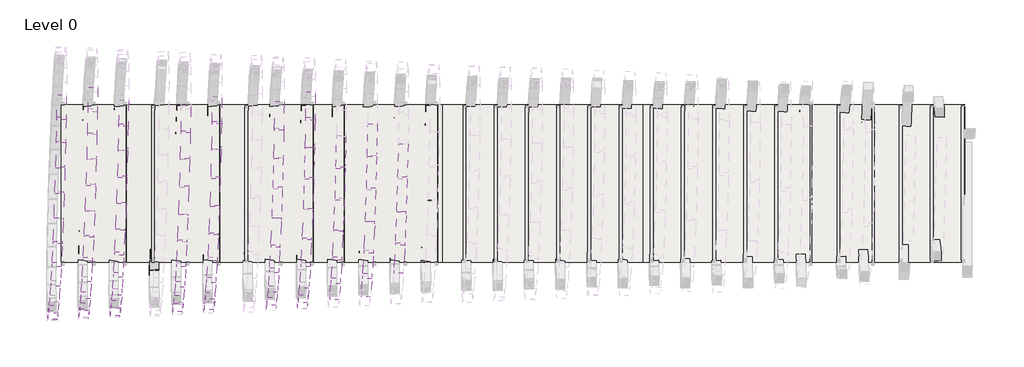
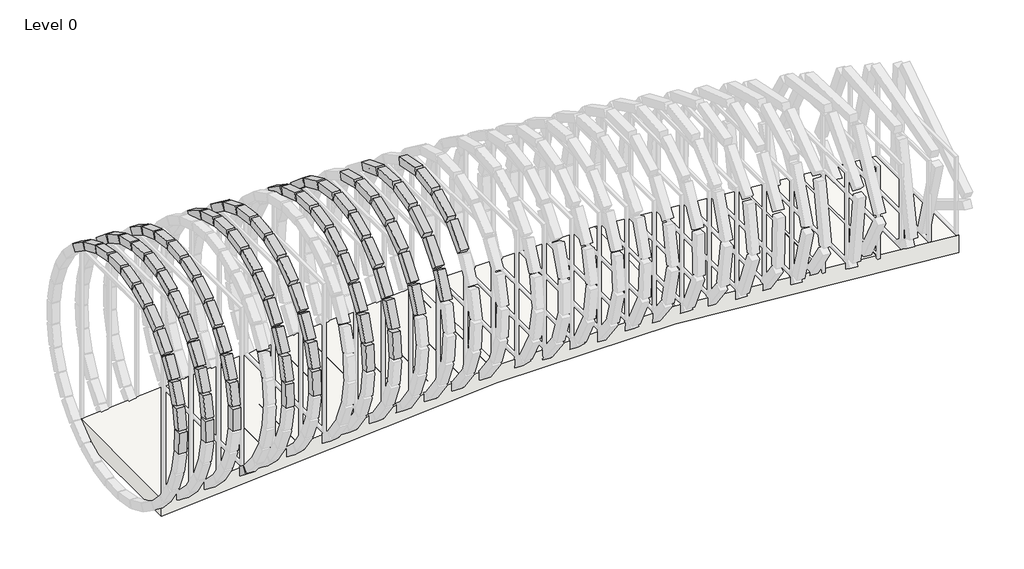
# One storey, part 1 of 6: 94 proxies, 1 slab.
"""IFC4 building model written with IfcOpenShell, lengths in millimetres."""

import ifcopenshell
import ifcopenshell.guid

model = None  # the IFC model being written
_history = None  # IfcOwnerHistory: only IFC2X3 demands one
_inside = {}  # id of a spatial element -> (the spatial element, [elements in it])
_under = {}  # id of a project, library or spatial element -> (it, [spatial elements below it])
_declared = {}  # id of a project -> (the project, [libraries it declares])
_typed = {}  # id of a type object -> (the type object, [elements of that type])
_made_of = {}  # id of a material, layer set ... -> (it, [elements and type objects made of it])


def new_model(schema):
    """Start an empty IFC model of exactly this schema.

    Asked for "IFC4X3", IfcOpenShell would pick the latest addendum, in which some entities
    have other attributes; the version numbers below select the first issue.
    IFC2X3 requires an IfcOwnerHistory on every rooted entity: one is made here for all.
    """
    global model, _history
    if schema == "IFC4X3":
        model = ifcopenshell.file(schema_version=(4, 3, 0, 0))
    else:
        model = ifcopenshell.file(schema=schema)
    _inside.clear()
    _under.clear()
    _declared.clear()
    _typed.clear()
    _made_of.clear()
    _history = None
    if model.schema == "IFC2X3":
        org = make("IfcOrganization", Name="unknown")
        user = make(
            "IfcPersonAndOrganization",
            ThePerson=make("IfcPerson", FamilyName="unknown"),
            TheOrganization=org,
        )
        app = make(
            "IfcApplication",
            ApplicationDeveloper=org,
            Version="unknown",
            ApplicationFullName="unknown",
            ApplicationIdentifier="unknown",
        )
        _history = make(
            "IfcOwnerHistory",
            OwningUser=user,
            OwningApplication=app,
            ChangeAction="ADDED",
            CreationDate=0,
        )
    return model


def make(cls, **values):
    """One entity of the class cls with the attributes given. An attribute that is None is left unset."""
    return model.create_entity(
        cls, **{name: value for name, value in values.items() if value is not None}
    )


def rooted(cls, **values):
    """An entity with a GlobalId (a new one), such as an element, a storey or a relation."""
    return make(cls, GlobalId=ifcopenshell.guid.new(), OwnerHistory=_history, **values)


def si_unit(unit_type, name, prefix=None):
    """IfcSIUnit, for example si_unit("LENGTHUNIT", "METRE", prefix="MILLI")."""
    return make("IfcSIUnit", UnitType=unit_type, Prefix=prefix, Name=name)


def assignment(units):
    """IfcUnitAssignment: the units of a project."""
    return None if units is None else make("IfcUnitAssignment", Units=units)


def point(xyz):
    """IfcCartesianPoint."""
    return None if xyz is None else make("IfcCartesianPoint", Coordinates=xyz)


def direction(xyz):
    """IfcDirection."""
    return None if xyz is None else make("IfcDirection", DirectionRatios=xyz)


def frame(location, z_axis=None, x_axis=None):
    """IfcAxis2Placement3D, a coordinate frame: its origin and axes. An axis left out is left unset."""
    return make(
        "IfcAxis2Placement3D",
        Location=point(location),
        Axis=direction(z_axis),
        RefDirection=direction(x_axis),
    )


def origin():
    """The frame at (0, 0, 0) with its axes left unset."""
    return frame((0.0, 0.0, 0.0))


def place(relative_to, where):
    """IfcLocalPlacement: puts the frame where relative to a parent placement (None: the world)."""
    return make(
        "IfcLocalPlacement", PlacementRelTo=relative_to, RelativePlacement=where
    )


def context(
    kind, dimensions, precision=None, world=None, true_north=None, identifier=None
):
    """IfcGeometricRepresentationContext, for example the 3D "Model" context."""
    return make(
        "IfcGeometricRepresentationContext",
        ContextIdentifier=identifier,
        ContextType=kind,
        CoordinateSpaceDimension=dimensions,
        Precision=precision,
        WorldCoordinateSystem=world,
        TrueNorth=true_north,
    )


def project(units=None, contexts=None):
    """IfcProject with its units and contexts."""
    return rooted(
        "IfcProject",
        Name="project",
        RepresentationContexts=contexts,
        UnitsInContext=assignment(units),
    )


def spatial(cls, under=None, at=None, **own):
    """A site, building, storey or space (cls), placed at a placement, below another one or the project."""
    s = rooted(cls, ObjectPlacement=at, **own)
    if under is not None:
        _under.setdefault(under.id(), (under, []))[1].append(s)
    return s


def polyline(points):
    """IfcPolyline through the points."""
    return make("IfcPolyline", Points=[point(p) for p in points])


def outline(outer, holes=None, kind="AREA"):
    """IfcArbitraryClosedProfileDef: a profile drawn as a closed curve; with holes, ...WithVoids."""
    if holes is None:
        return make("IfcArbitraryClosedProfileDef", ProfileType=kind, OuterCurve=outer)
    return make(
        "IfcArbitraryProfileDefWithVoids",
        ProfileType=kind,
        OuterCurve=outer,
        InnerCurves=holes,
    )


def extrude(swept, where, along, depth):
    """IfcExtrudedAreaSolid: the profile swept, set in the frame where, extruded along a direction by depth."""
    return make(
        "IfcExtrudedAreaSolid",
        SweptArea=swept,
        Position=where,
        ExtrudedDirection=direction(along),
        Depth=depth,
    )


def faces_of(points, faces, orient=None, outer=None):
    """IfcFace entities. A face is a list of loops; a loop is a list of indices into points, from 0.

    orient and outer hold one flag for each loop. By default every Orientation is true, the
    first loop of a face is its IfcFaceOuterBound and the others are IfcFaceBound.
    """
    made = []
    for i, loops in enumerate(faces):
        bounds = []
        for j, loop in enumerate(loops):
            is_outer = j == 0 if outer is None else outer[i][j]
            bounds.append(
                make(
                    "IfcFaceOuterBound" if is_outer else "IfcFaceBound",
                    Bound=make("IfcPolyLoop", Polygon=[points[k] for k in loop]),
                    Orientation=True if orient is None else orient[i][j],
                )
            )
        made.append(make("IfcFace", Bounds=bounds))
    return made


def faceted_brep(points, faces, orient=None, outer=None, voids=None):
    """IfcFacetedBrep: a solid bounded by flat faces; with voids (closed shells), ...WithVoids."""
    shared = [point(p) for p in points]
    hull = make("IfcClosedShell", CfsFaces=faces_of(shared, faces, orient, outer))
    if voids is None:
        return make("IfcFacetedBrep", Outer=hull)
    return make(
        "IfcFacetedBrepWithVoids",
        Outer=hull,
        Voids=[
            make(cls, CfsFaces=faces_of(shared, fs, o, b)) for cls, fs, o, b in voids
        ],
    )


def shape(context_of_items, identifier, shape_type, items):
    """IfcShapeRepresentation: the items that make up one representation, for example the "Body"."""
    return make(
        "IfcShapeRepresentation",
        ContextOfItems=context_of_items,
        RepresentationIdentifier=identifier,
        RepresentationType=shape_type,
        Items=items,
    )


def source(mapping_origin, context_of_items, identifier, shape_type, items):
    """IfcRepresentationMap: a shape defined once, which mapped items show again and again."""
    return make(
        "IfcRepresentationMap",
        MappingOrigin=mapping_origin,
        MappedRepresentation=shape(context_of_items, identifier, shape_type, items),
    )


def transform(
    local_origin,
    x_axis=None,
    y_axis=None,
    z_axis=None,
    scale=None,
    scale2=None,
    scale3=None,
    uniform=True,
):
    """IfcCartesianTransformationOperator3D, or its non-uniform kind. x_axis, y_axis, z_axis: its Axis1, 2, 3."""
    if uniform:
        return make(
            "IfcCartesianTransformationOperator3D",
            Axis1=direction(x_axis),
            Axis2=direction(y_axis),
            LocalOrigin=point(local_origin),
            Scale=scale,
            Axis3=direction(z_axis),
        )
    return make(
        "IfcCartesianTransformationOperator3DnonUniform",
        Axis1=direction(x_axis),
        Axis2=direction(y_axis),
        LocalOrigin=point(local_origin),
        Scale=scale,
        Axis3=direction(z_axis),
        Scale2=scale2,
        Scale3=scale3,
    )


def mapped(mapping_source, mapping_target):
    """IfcMappedItem: shows the shape of a source again, moved by a transform."""
    return make(
        "IfcMappedItem", MappingSource=mapping_source, MappingTarget=mapping_target
    )


def made_of(thing, what):
    """Note that an element or type object is made of a material, layer set ...; save() writes the relation."""
    if what is not None:
        _made_of.setdefault(what.id(), (what, []))[1].append(thing)
    return thing


def element(
    cls,
    number,
    at=None,
    inside=None,
    cuts=None,
    type_object=None,
    material=None,
    context=None,
    identifier="Body",
    shape_type=None,
    held_by="IfcProductDefinitionShape",
    body=None,
    shapes=None,
    **own,
):
    """One element of the class cls, such as IfcWall. Its Tag is "e" and its number.

    at: its placement. inside: the storey or other place that contains it. cuts: it is an
    opening in that element (IfcRelVoidsElement). A single representation is given by context,
    identifier, shape_type and body (its items); several are given by shapes. held_by: the class
    of the entity that holds the representations. save() writes the other relations.
    """
    e = rooted(cls, Tag="e%d" % number, ObjectPlacement=at, **own)
    if body is not None:
        shapes = [shape(context, identifier, shape_type, body)]
    if shapes is not None:
        e.Representation = make(held_by, Representations=shapes)
    if inside is not None:
        _inside.setdefault(inside.id(), (inside, []))[1].append(e)
    if cuts is not None:
        rooted(
            "IfcRelVoidsElement", RelatingBuildingElement=cuts, RelatedOpeningElement=e
        )
    if type_object is not None:
        _typed.setdefault(type_object.id(), (type_object, []))[1].append(e)
    return made_of(e, material)


def aggregate(whole, parts):
    """IfcRelAggregates: a whole, such as a stair, and the parts it consists of."""
    return rooted("IfcRelAggregates", RelatingObject=whole, RelatedObjects=parts)


def save(model, path):
    """Write the relations noted so far, then the file.

    IfcRelAggregates (storeys below a building ...), IfcRelContainedInSpatialStructure (elements
    in a storey), IfcRelDefinesByType, IfcRelAssociatesMaterial and IfcRelDeclares: one each for
    every whole, place, type object, material and project.
    """
    for whole, parts in _under.values():
        aggregate(whole, parts)
    for where, things in _inside.values():
        rooted(
            "IfcRelContainedInSpatialStructure",
            RelatedElements=things,
            RelatingStructure=where,
        )
    for kind, things in _typed.values():
        rooted("IfcRelDefinesByType", RelatedObjects=things, RelatingType=kind)
    for what, things in _made_of.values():
        rooted("IfcRelAssociatesMaterial", RelatedObjects=things, RelatingMaterial=what)
    for by, libraries in _declared.values():
        rooted("IfcRelDeclares", RelatingContext=by, RelatedDefinitions=libraries)
    model.write(path)


def family2_family2_c0c01265(model_context):
    return source(origin(), model_context, "Body", "Brep", [
        faceted_brep([(-3947.6024006, -6432.4470029, 1.0945136), (-3947.6024006, -6432.4470029, 201.0945136), (-3939.2403939, -5715.1531197, 202.060409), (-3939.2403939, -5715.1531197, 2.060409), (-3747.6112106, -6434.3242155, 201.0945136), (-3739.249204, -5717.0303324, 202.060409), (-3747.6112106, -6434.3242155, 1.0945136), (-3739.249204, -5717.0303324, 2.060409)], [[[0, 1, 2, 3]], [[1, 4, 5, 2]], [[4, 6, 7, 5]], [[6, 0, 3, 7]], [[3, 2, 5, 7]], [[0, 6, 4, 1]]]),
    ])


def family2_family2_390b1421(model_context):
    return source(origin(), model_context, "Body", "Brep", [
        faceted_brep([(-3947.4886476, -6420.3281868, 1.0945136), (-3947.4886476, -6420.3281868, 201.0945136), (-3939.3541469, -5727.2719358, 202.060409), (-3939.3541469, -5727.2719358, 2.060409), (-3747.4974576, -6422.2053995, 201.0945136), (-3739.3629569, -5729.1491484, 202.060409), (-3747.4974576, -6422.2053995, 1.0945136), (-3739.3629569, -5729.1491484, 2.060409)], [[[0, 1, 2, 3]], [[1, 4, 5, 2]], [[4, 6, 7, 5]], [[6, 0, 3, 7]], [[3, 2, 5, 7]], [[0, 6, 4, 1]]]),
    ])


def family2_family2_5d0bf995(model_context):
    return source(origin(), model_context, "Body", "Brep", [
        faceted_brep([(-3947.3850716, -6409.2935888, 1.0945136), (-3947.3850716, -6409.2935888, 201.0945136), (-3939.4577229, -5738.3065338, 202.060409), (-3939.4577229, -5738.3065338, 2.060409), (-3747.3938816, -6411.1708015, 201.0945136), (-3739.4665329, -5740.1837465, 202.060409), (-3747.3938816, -6411.1708015, 1.0945136), (-3739.4665329, -5740.1837465, 2.060409)], [[[0, 1, 2, 3]], [[1, 4, 5, 2]], [[4, 6, 7, 5]], [[6, 0, 3, 7]], [[3, 2, 5, 7]], [[0, 6, 4, 1]]]),
    ])


def family2_family2_428b8be4(model_context):
    return source(origin(), model_context, "Body", "Brep", [
        faceted_brep([(-3947.2904042, -6399.2080776, 1.0945136), (-3947.2904042, -6399.2080776, 201.0945136), (-3939.5523903, -5748.392045, 202.060409), (-3939.5523903, -5748.392045, 2.060409), (-3747.2992142, -6401.0852903, 201.0945136), (-3739.5612004, -5750.2692577, 202.060409), (-3747.2992142, -6401.0852903, 1.0945136), (-3739.5612004, -5750.2692577, 2.060409)], [[[0, 1, 2, 3]], [[1, 4, 5, 2]], [[4, 6, 7, 5]], [[6, 0, 3, 7]], [[3, 2, 5, 7]], [[0, 6, 4, 1]]]),
    ])


def family2_family2_042d18f2(model_context):
    return source(origin(), model_context, "Body", "Brep", [
        faceted_brep([(-3947.2035772, -6389.957857, 1.0945136), (-3947.2035772, -6389.957857, 201.0945136), (-3939.6392173, -5757.6422656, 202.060409), (-3939.6392173, -5757.6422656, 2.060409), (-3747.2123872, -6391.8350697, 201.0945136), (-3739.6480273, -5759.5194783, 202.060409), (-3747.2123872, -6391.8350697, 1.0945136), (-3739.6480273, -5759.5194783, 2.060409)], [[[0, 1, 2, 3]], [[1, 4, 5, 2]], [[4, 6, 7, 5]], [[6, 0, 3, 7]], [[3, 2, 5, 7]], [[0, 6, 4, 1]]]),
    ])


def family2_family2_49637704(model_context):
    return source(origin(), model_context, "Body", "Brep", [
        faceted_brep([(-3947.1236849, -6381.446434, 1.0945136), (-3947.1236849, -6381.446434, 201.0945136), (-3939.7191096, -5766.1536886, 202.060409), (-3939.7191096, -5766.1536886, 2.060409), (-3747.1324949, -6383.3236466, 201.0945136), (-3739.7279196, -5768.0309013, 202.060409), (-3747.1324949, -6383.3236466, 1.0945136), (-3739.7279196, -5768.0309013, 2.060409)], [[[0, 1, 2, 3]], [[1, 4, 5, 2]], [[4, 6, 7, 5]], [[6, 0, 3, 7]], [[3, 2, 5, 7]], [[0, 6, 4, 1]]]),
    ])


def family2_family2_4fb73a58(model_context):
    return source(origin(), model_context, "Body", "Brep", [
        faceted_brep([(-3947.0499544, -6373.591465, 1.0945136), (-3947.0499544, -6373.591465, 201.0945136), (-3939.7928401, -5774.0086576, 202.060409), (-3939.7928401, -5774.0086576, 2.060409), (-3747.0587644, -6375.4686776, 201.0945136), (-3739.8016501, -5775.8858703, 202.060409), (-3747.0587644, -6375.4686776, 1.0945136), (-3739.8016501, -5775.8858703, 2.060409)], [[[0, 1, 2, 3]], [[1, 4, 5, 2]], [[4, 6, 7, 5]], [[6, 0, 3, 7]], [[3, 2, 5, 7]], [[0, 6, 4, 1]]]),
    ])


def family2_family2_6873a2fb(model_context):
    return source(origin(), model_context, "Body", "Brep", [
        faceted_brep([(-3946.9817223, -6366.3222661, 1.0945136), (-3946.9817223, -6366.3222661, 201.0945136), (-3939.8610722, -5781.2778565, 202.060409), (-3939.8610722, -5781.2778565, 2.060409), (-3746.9905323, -6368.1994787, 201.0945136), (-3739.8698823, -5783.1550692, 202.060409), (-3746.9905323, -6368.1994787, 1.0945136), (-3739.8698823, -5783.1550692, 2.060409)], [[[0, 1, 2, 3]], [[1, 4, 5, 2]], [[4, 6, 7, 5]], [[6, 0, 3, 7]], [[3, 2, 5, 7]], [[0, 6, 4, 1]]]),
    ])


def family2_family2_2698309a(model_context):
    return source(origin(), model_context, "Body", "Brep", [
        faceted_brep([(-3946.9184158, -6359.5778294, 1.0945136), (-3946.9184158, -6359.5778294, 201.0945136), (-3939.9243787, -5788.0222932, 202.060409), (-3939.9243787, -5788.0222932, 2.060409), (-3746.9272258, -6361.4550421, 201.0945136), (-3739.9331888, -5789.8995058, 202.060409), (-3746.9272258, -6361.4550421, 1.0945136), (-3739.9331888, -5789.8995058, 2.060409)], [[[0, 1, 2, 3]], [[1, 4, 5, 2]], [[4, 6, 7, 5]], [[6, 0, 3, 7]], [[3, 2, 5, 7]], [[0, 6, 4, 1]]]),
    ])


def family2_family2_b00769dc(model_context):
    return source(origin(), model_context, "Body", "Brep", [
        faceted_brep([(-3946.8595382, -6353.3052302, 1.0945136), (-3946.8595382, -6353.3052302, 201.0945136), (-3939.9832564, -5794.2948924, 202.060409), (-3939.9832564, -5794.2948924, 2.060409), (-3746.8683482, -6355.1824428, 201.0945136), (-3739.9920664, -5796.1721051, 202.060409), (-3746.8683482, -6355.1824428, 1.0945136), (-3739.9920664, -5796.1721051, 2.060409)], [[[0, 1, 2, 3]], [[1, 4, 5, 2]], [[4, 6, 7, 5]], [[6, 0, 3, 7]], [[3, 2, 5, 7]], [[0, 6, 4, 1]]]),
    ])


def family2_family2_2f13623d(model_context):
    return source(origin(), model_context, "Body", "Brep", [
        faceted_brep([(-3946.8046564, -6347.4583376, 1.0945136), (-3946.8046564, -6347.4583376, 201.0945136), (-3940.0381381, -5800.141785, 202.060409), (-3940.0381381, -5800.141785, 2.060409), (-3746.8134664, -6349.3355503, 201.0945136), (-3740.0469481, -5802.0189977, 202.060409), (-3746.8134664, -6349.3355503, 1.0945136), (-3740.0469481, -5802.0189977, 2.060409)], [[[0, 1, 2, 3]], [[1, 4, 5, 2]], [[4, 6, 7, 5]], [[6, 0, 3, 7]], [[3, 2, 5, 7]], [[0, 6, 4, 1]]]),
    ])


def family2_family2_c4a0287a(model_context):
    return source(origin(), model_context, "Body", "Brep", [
        faceted_brep([(-3946.7533915, -6341.9967642, 1.0945136), (-3946.7533915, -6341.9967642, 201.0945136), (-3940.089403, -5805.6033584, 202.060409), (-3940.089403, -5805.6033584, 2.060409), (-3746.7622015, -6343.8739769, 201.0945136), (-3740.098213, -5807.480571, 202.060409), (-3746.7622015, -6343.8739769, 1.0945136), (-3740.098213, -5807.480571, 2.060409)], [[[0, 1, 2, 3]], [[1, 4, 5, 2]], [[4, 6, 7, 5]], [[6, 0, 3, 7]], [[3, 2, 5, 7]], [[0, 6, 4, 1]]]),
    ])


model = new_model("IFC4")

# Units and contexts
model_context = context("Model", 3, world=origin())
ifc_project = project(units=[si_unit("LENGTHUNIT", "METRE", prefix="MILLI")], contexts=[model_context])

# Site, building, storey
site = spatial("IfcSite", under=ifc_project)
building = spatial("IfcBuilding", under=site)
storey = spatial("IfcBuildingStorey", under=building, Name="Level 0", Elevation=0.0)

# Proxies
placement = place(None, origin())
family2_family2_shape = family2_family2_c0c01265(model_context)
element("IfcBuildingElementProxy", 1, Name="Family2 : Family2", ObjectType="Family2 : Family2", at=placement, inside=storey, context=model_context, shape_type="MappedRepresentation", body=[
    mapped(family2_family2_shape, transform((-6396.5684291, -2837.5092631, 6085.2878101), x_axis=(-0.9993635970569693, 0.019515115875459933, 0.029859020910323705), y_axis=(-0.013210966255060963, -0.9800389734063266, 0.1983660277751243), z_axis=(0.03313414021765793, 0.19784532053359544, 0.9796730872566602))),
])
element("IfcBuildingElementProxy", 2, Name="Family2 : Family2", ObjectType="Family2 : Family2", at=placement, inside=storey, context=model_context, shape_type="MappedRepresentation", body=[
    mapped(family2_family2_shape, transform((-6470.2682928, -3665.5268728, 4304.1033014), x_axis=(-0.9994458455142355, 0.019376337243089063, 0.02706583527950426), y_axis=(-0.021973408141946323, -0.9948239279417687, -0.09920948406850226), z_axis=(0.025003424144757144, -0.09974923533317458, 0.994698405966092))),
])
element("IfcBuildingElementProxy", 3, Name="Family2 : Family2", ObjectType="Family2 : Family2", at=placement, inside=storey, context=model_context, shape_type="MappedRepresentation", body=[
    mapped(family2_family2_shape, transform((-6532.4519203, -3931.5588011, 2357.5619339), x_axis=(-0.999501945539641, 0.020067046494086277, 0.02435517414179686), y_axis=(-0.02795009425626786, -0.9212383571752715, -0.3879931462024461), z_axis=(0.014651044110875288, -0.38848063389828225, 0.9213404061433809))),
])
element("IfcBuildingElementProxy", 4, Name="Family2 : Family2", ObjectType="Family2 : Family2", at=placement, inside=storey, context=model_context, shape_type="MappedRepresentation", body=[
    mapped(family2_family2_shape, transform((-6577.5940234, -3611.9669438, 418.6224503), x_axis=(-0.9995269123997371, 0.02152587108037278, 0.021967891634827073), y_axis=(-0.030609969808513042, -0.7658206619943964, -0.6423252629398807), z_axis=(0.002996854512694002, -0.6426938233223469, 0.7661172679990537))),
])
family2_family2_2_shape = family2_family2_390b1421(model_context)
element("IfcBuildingElementProxy", 5, Name="Family2 : Family2", ObjectType="Family2 : Family2", at=placement, inside=storey, context=model_context, shape_type="MappedRepresentation", body=[
    mapped(family2_family2_2_shape, transform((-7043.8373064, -2077.9606819, 7037.3849212), x_axis=(-0.9993079250855319, 0.020318015980282017, 0.03115845130738213), y_axis=(-0.007279883403612856, -0.9282706726012948, 0.371834051272836), z_axis=(0.03647840674809277, 0.3713498843610499, 0.92777615254228))),
])
element("IfcBuildingElementProxy", 6, Name="Family2 : Family2", ObjectType="Family2 : Family2", at=placement, inside=storey, context=model_context, shape_type="MappedRepresentation", body=[
    mapped(family2_family2_2_shape, transform((-7118.0067992, -3181.769788, 5516.9346303), x_axis=(-0.9993980532845504, 0.019688875205587705, 0.028563600686710367), y_axis=(-0.016881803397264153, -0.9952969690227281, 0.09538840688588489), z_axis=(0.03030735562709434, 0.09484878305655688, 0.9950302370016618))),
])
element("IfcBuildingElementProxy", 7, Name="Family2 : Family2", ObjectType="Family2 : Family2", at=placement, inside=storey, context=model_context, shape_type="MappedRepresentation", body=[
    mapped(family2_family2_2_shape, transform((-7185.3404976, -3812.2729758, 3746.7378484), x_axis=(-0.9994682121798837, 0.019816387397900603, 0.025896015763889266), y_axis=(-0.0243562687384851, -0.9817122987182729, -0.18880607701666632), z_axis=(0.02168098279797224, -0.18933640256374623, 0.9816728893318453))),
])
element("IfcBuildingElementProxy", 8, Name="Family2 : Family2", ObjectType="Family2 : Family2", at=placement, inside=storey, context=model_context, shape_type="MappedRepresentation", body=[
    mapped(family2_family2_2_shape, transform((-7240.3834258, -3918.3906269, 1870.205391), x_axis=(-0.9995127179150824, 0.020690222277743867, 0.02337180840462852), y_axis=(-0.029097742697687057, -0.8886172108848517, -0.457725653518706), z_axis=(0.011298145684328523, -0.45818267887527653, 0.8887862424018338))),
])
element("IfcBuildingElementProxy", 9, Name="Family2 : Family2", ObjectType="Family2 : Family2", at=placement, inside=storey, context=model_context, shape_type="MappedRepresentation", body=[
    mapped(family2_family2_2_shape, transform((-7278.6763332, -3491.5257202, 39.3627577), x_axis=(-0.9995279649001668, 0.02223958694004874, 0.021195474877135474), y_axis=(-0.030722099253326866, -0.7235537158809213, -0.6895840578583441), z_axis=(0.0, -0.6899097194616461, 0.7238954199277359))),
])
element("IfcBuildingElementProxy", 10, Name="Family2 : Family2", ObjectType="Family2 : Family2", at=placement, inside=storey, context=model_context, shape_type="MappedRepresentation", body=[
    mapped(family2_family2_2_shape, transform((-7297.1169561, -2566.2603118, -1597.4660699), x_axis=(-0.9995127179150824, 0.02433896107430176, 0.019543328780653933), y_axis=(-0.029097742697686946, -0.49989427640129913, -0.8655975010310053), z_axis=(-0.011298145684328832, -0.865744377628319, 0.5003588957029249))),
])
family2_family2_3_shape = family2_family2_5d0bf995(model_context)
element("IfcBuildingElementProxy", 11, Name="Family2 : Family2", ObjectType="Family2 : Family2", at=placement, inside=storey, context=model_context, shape_type="MappedRepresentation", body=[
    mapped(family2_family2_3_shape, transform((-7766.7940735, -2531.5035471, 6528.1339417), x_axis=(-0.9993471346343662, 0.020301994662961675, 0.02988533939555133), y_axis=(-0.011457121548771567, -0.9625718139560835, 0.27078448504874103), z_axis=(0.03426425052294141, 0.27026529927092063, 0.9621759865773523))),
])
element("IfcBuildingElementProxy", 12, Name="Family2 : Family2", ObjectType="Family2 : Family2", at=placement, inside=storey, context=model_context, shape_type="MappedRepresentation", body=[
    mapped(family2_family2_3_shape, transform((-7836.0862349, -3444.6813187, 4975.6904694), x_axis=(-0.9994266506244945, 0.019952546178124225, 0.027354449775399966), y_axis=(-0.019928456644108153, -0.9998007437454588, 0.0011530055558309493), z_axis=(0.027372004626789022, 0.0006072125144431367, 0.9996251320648525))),
])
element("IfcBuildingElementProxy", 13, Name="Family2 : Family2", ObjectType="Family2 : Family2", at=placement, inside=storey, context=model_context, shape_type="MappedRepresentation", body=[
    mapped(family2_family2_3_shape, transform((-7897.2581176, -3904.9775123, 3234.0931577), x_axis=(-0.9994857645079068, 0.02029891933854758, 0.024822578829211326), y_axis=(-0.02622622787686343, -0.9628994474747761, -0.2685830207293869), z_axis=(0.01844970236605738, -0.2690959084164204, 0.9629366544877943))),
])
element("IfcBuildingElementProxy", 14, Name="Family2 : Family2", ObjectType="Family2 : Family2", at=placement, inside=storey, context=model_context, shape_type="MappedRepresentation", body=[
    mapped(family2_family2_3_shape, transform((-7945.772883, -3878.254065, 1432.5083121), x_axis=(-0.9995200920782988, 0.02131542523147494, 0.022477503842524255), y_axis=(-0.02988335836509007, -0.8546047254762345, -0.5184185066975466), z_axis=(0.008159070082607002, -0.5188414168519047, 0.8548315703894513))),
])
element("IfcBuildingElementProxy", 15, Name="Family2 : Family2", ObjectType="Family2 : Family2", at=placement, inside=storey, context=model_context, shape_type="MappedRepresentation", body=[
    mapped(family2_family2_3_shape, transform((-7978.0324128, -3366.4929326, -295.4487611), x_axis=(-0.9995270874168127, 0.022926674265032795, 0.02049314829909779), y_axis=(-0.03062861547073516, -0.6829483018650779, -0.7298242972756885), z_axis=(-0.002736683103608129, -0.7301068309410284, 0.6833275393095458))),
])
element("IfcBuildingElementProxy", 16, Name="Family2 : Family2", ObjectType="Family2 : Family2", at=placement, inside=storey, context=model_context, shape_type="MappedRepresentation", body=[
    mapped(family2_family2_3_shape, transform((-7991.6441653, -2407.6490971, -1821.6233908), x_axis=(-0.999506231711192, 0.025013167469376377, 0.019016682771764888), y_axis=(-0.02840672688359737, -0.46066114830466015, -0.8871213920937727), z_axis=(-0.013429469023521176, -0.887223561395763, 0.46114423065453763))),
])
family2_family2_4_shape = family2_family2_428b8be4(model_context)
element("IfcBuildingElementProxy", 17, Name="Family2 : Family2", ObjectType="Family2 : Family2", at=placement, inside=storey, context=model_context, shape_type="MappedRepresentation", body=[
    mapped(family2_family2_4_shape, transform((-8349.1757108, -349.9613425, 8322.8659908), x_axis=(-0.9992006919462781, 0.022454860439543138, 0.033071989004595945), y_axis=(0.0041443327129058564, -0.7646748671158883, 0.6444029578669418), z_axis=(0.03975929728307849, 0.644024942718789, 0.7639705959234404))),
])
element("IfcBuildingElementProxy", 18, Name="Family2 : Family2", ObjectType="Family2 : Family2", at=placement, inside=storey, context=model_context, shape_type="MappedRepresentation", body=[
    mapped(family2_family2_4_shape, transform((-8417.9429112, -1775.2827593, 7343.0038201), x_axis=(-0.9992956048051683, 0.021134817771098994, 0.03100989672435847), y_axis=(-0.005967326982465977, -0.9053072577395126, 0.42471538716280155), z_axis=(0.037049766878582024, 0.4242311734914662, 0.9047956820256695))),
])
element("IfcBuildingElementProxy", 19, Name="Family2 : Family2", ObjectType="Family2 : Family2", at=placement, inside=storey, context=model_context, shape_type="MappedRepresentation", body=[
    mapped(family2_family2_4_shape, transform((-8486.820728, -2898.1535958, 6027.3986842), x_axis=(-0.9993807013464429, 0.020393697698042258, 0.028675963287971513), y_axis=(-0.015033193048246478, -0.9842634082524215, 0.17606688013962607), z_axis=(0.03181535608894513, 0.17552675086586705, 0.9839604376434075))),
])
element("IfcBuildingElementProxy", 20, Name="Family2 : Family2", ObjectType="Family2 : Family2", at=placement, inside=storey, context=model_context, shape_type="MappedRepresentation", body=[
    mapped(family2_family2_4_shape, transform((-8551.115252, -3642.0520602, 4465.7068992), x_axis=(-0.9994501823814422, 0.020282006328592724, 0.02622924240211747), y_axis=(-0.022435441694104982, -0.9961625874783727, -0.08459757836004667), z_axis=(0.024412781359208695, -0.08513952975957023, 0.9960699155072533))),
])
element("IfcBuildingElementProxy", 21, Name="Family2 : Family2", ObjectType="Family2 : Family2", at=placement, inside=storey, context=model_context, shape_type="MappedRepresentation", body=[
    mapped(family2_family2_4_shape, transform((-8606.4449175, -3956.2827014, 2764.3551793), x_axis=(-0.9994993128924541, 0.020807355244999624, 0.023836474051769297), y_axis=(-0.02766962190762047, -0.9401938860174409, -0.33951413625784876), z_axis=(0.015346515923870596, -0.3400036921316182, 0.940298874712645))),
])
element("IfcBuildingElementProxy", 22, Name="Family2 : Family2", ObjectType="Family2 : Family2", at=placement, inside=storey, context=model_context, shape_type="MappedRepresentation", body=[
    mapped(family2_family2_4_shape, transform((-8649.0390993, -3819.4312207, 1039.2878327), x_axis=(-0.9995247447163452, 0.021933942786790245, 0.021660721445766612), y_axis=(-0.030379032957133623, -0.820171478381537, -0.5713106514025741), z_axis=(0.005234410789637128, -0.571697164767563, 0.8204480195237328))),
])
element("IfcBuildingElementProxy", 23, Name="Family2 : Family2", ObjectType="Family2 : Family2", at=placement, inside=storey, context=model_context, shape_type="MappedRepresentation", body=[
    mapped(family2_family2_4_shape, transform((-8675.9950743, -3240.8238202, -591.9346519), x_axis=(-0.9995247447163452, 0.023584993874764825, 0.019850258528608347), y_axis=(-0.03037903295713377, -0.6442746933046386, -0.7641905743489666), z_axis=(-0.005234410789636466, -0.7644304203988362, 0.6446849876587355))),
])
element("IfcBuildingElementProxy", 24, Name="Family2 : Family2", ObjectType="Family2 : Family2", at=placement, inside=storey, context=model_context, shape_type="MappedRepresentation", body=[
    mapped(family2_family2_4_shape, transform((-8685.4758373, -2259.8916381, -2018.1471577), x_axis=(-0.9994993128924541, 0.025647992105770276, 0.018528465356165688), y_axis=(-0.027669621907620588, -0.42449060600655897, -0.9050094570973686), z_axis=(-0.015346515923870454, -0.9050690061609262, 0.42498773927711336))),
])
element("IfcBuildingElementProxy", 25, Name="Family2 : Family2", ObjectType="Family2 : Family2", at=placement, inside=storey, context=model_context, shape_type="MappedRepresentation", body=[
    mapped(family2_family2_4_shape, transform((-8676.83529, -943.4835816, -3142.1556595), x_axis=(-0.9994501823814423, 0.02798234755962721, 0.01778541994877588), y_axis=(-0.022435441694105274, -0.17579713882628062, -0.9841707255026864), z_axis=(-0.024412781359207977, -0.9840286348504019, 0.1763282787892001))),
])
family2_family2_5_shape = family2_family2_042d18f2(model_context)
element("IfcBuildingElementProxy", 26, Name="Family2 : Family2", ObjectType="Family2 : Family2", at=placement, inside=storey, context=model_context, shape_type="MappedRepresentation", body=[
    mapped(family2_family2_5_shape, transform((-9072.2091725, -959.7625262, 7975.489109), x_axis=(-0.9992451691704809, 0.022120695462552988, 0.031933786523220827), y_axis=(-0.0005941037918020704, -0.8306451189080555, 0.5568018799132303), z_axis=(0.03884248872230278, 0.5563626167046775, 0.8300312643529654))),
])
element("IfcBuildingElementProxy", 27, Name="Family2 : Family2", ObjectType="Family2 : Family2", at=placement, inside=storey, context=model_context, shape_type="MappedRepresentation", body=[
    mapped(family2_family2_5_shape, transform((-9138.9684474, -2229.7814255, 6900.4046938), x_axis=(-0.9993328951874266, 0.02106689224108586, 0.029832040621093254), y_axis=(-0.009940104324900365, -0.9429133582798052, 0.3328897611875592), z_axis=(0.03514198233347372, 0.33237115522981625, 0.9424937433473346))),
])
element("IfcBuildingElementProxy", 28, Name="Family2 : Family2", ObjectType="Family2 : Family2", at=placement, inside=storey, context=model_context, shape_type="MappedRepresentation", body=[
    mapped(family2_family2_5_shape, transform((-9204.0667907, -3192.3094108, 5543.0125661), x_axis=(-0.9994092273378256, 0.02056904131601685, 0.027533812873467303), y_axis=(-0.018072245087193965, -0.9959525269675568, 0.0880452042103769), z_axis=(0.02923337595146198, 0.08749559169625962, 0.9957358741976721))),
])
element("IfcBuildingElementProxy", 29, Name="Family2 : Family2", ObjectType="Family2 : Family2", at=placement, inside=storey, context=model_context, shape_type="MappedRepresentation", body=[
    mapped(family2_family2_5_shape, transform((-9263.4138341, -3786.8673088, 3988.6026654), x_axis=(-0.9994693693919375, 0.020658424491935765, 0.025183509382017088), y_axis=(-0.024479553766666155, -0.9864299789382394, -0.16234730702814268), z_axis=(0.02148792904558406, -0.1628776416498474, 0.986412258011789))),
])
element("IfcBuildingElementProxy", 30, Name="Family2 : Family2", ObjectType="Family2 : Family2", at=placement, inside=storey, context=model_context, shape_type="MappedRepresentation", body=[
    mapped(family2_family2_5_shape, transform((-9313.2805845, -3976.0968602, 2334.8442825), x_axis=(-0.999509542403316, 0.021329425495171216, 0.022928808358921703), y_axis=(-0.028759435594552796, -0.914944050906018, -0.40255469016764567), z_axis=(0.012392316530697053, -0.4030166737490303, 0.9151087318845073))),
])
element("IfcBuildingElementProxy", 31, Name="Family2 : Family2", ObjectType="Family2 : Family2", at=placement, inside=storey, context=model_context, shape_type="MappedRepresentation", body=[
    mapped(family2_family2_5_shape, transform((-9350.5337307, -3748.1080763, 685.6491386), x_axis=(-0.9995272221539101, 0.02253988286492099, 0.02091138096167241), y_axis=(-0.03064296985530348, -0.785986466636009, -0.6174838319045202), z_axis=(0.0025180491924339486, -0.6178326860449179, 0.7863055585984284))),
])
element("IfcBuildingElementProxy", 32, Name="Family2 : Family2", ObjectType="Family2 : Family2", at=placement, inside=storey, context=model_context, shape_type="MappedRepresentation", body=[
    mapped(family2_family2_5_shape, transform((-9372.8325204, -3117.2263309, -855.35777), x_axis=(-0.9995212977599682, 0.024213739112893127, 0.019257989573217338), y_axis=(-0.030011807164160687, -0.6076601054207175, -0.793629943809345), z_axis=(-0.007514436437327189, -0.7938279984469279, 0.6080959152360539))),
])
element("IfcBuildingElementProxy", 33, Name="Family2 : Family2", ObjectType="Family2 : Family2", at=placement, inside=storey, context=model_context, shape_type="MappedRepresentation", body=[
    mapped(family2_family2_5_shape, transform((-9378.7758387, -2123.0922443, -2191.3493119), x_axis=(-0.9994921414729501, 0.026245819695013738, 0.018072522855242232), y_axis=(-0.026905605794263134, -0.39116986837377654, -0.9199251178510598), z_axis=(-0.01707476238956601, -0.9199441782113627, 0.39167736909905915))),
])
element("IfcBuildingElementProxy", 34, Name="Family2 : Family2", ObjectType="Family2 : Family2", at=placement, inside=storey, context=model_context, shape_type="MappedRepresentation", body=[
    mapped(family2_family2_5_shape, transform((-9367.9902451, -828.1709173, -3238.3802249), x_axis=(-0.9994415852895988, 0.02850844151484034, 0.017429468041477797), y_axis=(-0.0215195398014908, -0.15011863328424735, -0.9884337637634611), z_axis=(-0.025562218224286025, -0.9882568819407559, 0.15064829337297314))),
])
family2_family2_6_shape = family2_family2_49637704(model_context)
element("IfcBuildingElementProxy", 35, Name="Family2 : Family2", ObjectType="Family2 : Family2", at=placement, inside=storey, context=model_context, shape_type="MappedRepresentation", body=[
    mapped(family2_family2_6_shape, transform((-2219.5497597, -4200.7890895, 2742.0107907), x_axis=(0.9990180869271126, -0.03847010902675502, -0.021975274832456145), y_axis=(-0.023598385978757203, -0.8818420404359023, 0.4709540655934956), z_axis=(-0.03749637544736816, -0.4699730486222741, -0.8818839806896345))),
])
element("IfcBuildingElementProxy", 36, Name="Family2 : Family2", ObjectType="Family2 : Family2", at=placement, inside=storey, context=model_context, shape_type="MappedRepresentation", body=[
    mapped(family2_family2_6_shape, transform((-2259.9991266, -4138.1407116, 1139.1037078), x_axis=(0.9989377398963087, -0.03928517431786254, -0.024084577838741083), y_axis=(-0.032158257028073775, -0.9686760368989771, 0.24623684135930654), z_axis=(-0.03300361064749686, -0.2452007557421206, -0.9689103937246837))),
])
family2_family2_7_shape = family2_family2_4fb73a58(model_context)
element("IfcBuildingElementProxy", 37, Name="Family2 : Family2", ObjectType="Family2 : Family2", at=placement, inside=storey, context=model_context, shape_type="MappedRepresentation", body=[
    mapped(family2_family2_7_shape, transform((-10450.7209705, -699.1211328, 8147.4677295), x_axis=(-0.9992383660480748, 0.02287178206474072, 0.03161596752840712), y_axis=(0.00013067533128338117, -0.8082505413987439, 0.5888387260129853), z_axis=(0.03902141388432872, 0.5883943778740758, 0.8076319615670539))),
])
element("IfcBuildingElementProxy", 38, Name="Family2 : Family2", ObjectType="Family2 : Family2", at=placement, inside=storey, context=model_context, shape_type="MappedRepresentation", body=[
    mapped(family2_family2_7_shape, transform((-10512.6953237, -1935.4535094, 7217.1654775), x_axis=(-0.9993204910017381, 0.021802584337080023, 0.029718741229564), y_axis=(-0.008618608945386646, -0.9221588536713061, 0.38671535808068114), z_axis=(0.03583679455380706, 0.38619644730609237, 0.9217201463808093))),
])
element("IfcBuildingElementProxy", 39, Name="Family2 : Family2", ObjectType="Family2 : Family2", at=placement, inside=storey, context=model_context, shape_type="MappedRepresentation", body=[
    mapped(family2_family2_7_shape, transform((-10573.9028849, -2923.7176536, 6026.6158307), x_axis=(-0.9993935089187473, 0.021199879590631188, 0.027625702460149778), y_axis=(-0.016397663723566148, -0.9863687548809619, 0.1637308645887826), z_axis=(0.03072020435288198, 0.16317856630061484, 0.9861181595248071))),
])
element("IfcBuildingElementProxy", 40, Name="Family2 : Family2", ObjectType="Family2 : Family2", at=placement, inside=storey, context=model_context, shape_type="MappedRepresentation", body=[
    mapped(family2_family2_7_shape, transform((-10631.0439387, -3610.6359896, 4640.0016286), x_axis=(-0.9994534833842964, 0.02109615979427901, 0.025449687481984846), y_axis=(-0.022787118146630203, -0.9974186726333861, -0.0680936027011809), z_axis=(0.023947479983663554, -0.0686363134513284, 0.9973542874416508))),
])
element("IfcBuildingElementProxy", 41, Name="Family2 : Family2", ObjectType="Family2 : Family2", at=placement, inside=storey, context=model_context, shape_type="MappedRepresentation", body=[
    mapped(family2_family2_7_shape, transform((-10681.0379961, -3959.176572, 3132.0756017), x_axis=(-0.9994971811594235, 0.021497016509091856, 0.023308005825784555), y_axis=(-0.02744251507278282, -0.9547129030023807, -0.2962603267520766), z_axis=(0.01588374076995283, -0.2967509917792609, 0.9548227875669798))),
])
element("IfcBuildingElementProxy", 42, Name="Family2 : Family2", ObjectType="Family2 : Family2", at=placement, inside=storey, context=model_context, shape_type="MappedRepresentation", body=[
    mapped(family2_family2_7_shape, transform((-10721.1898645, -3950.549488, 1584.1304325), x_axis=(-0.999522246485761, 0.022380839445816363, 0.02131611610398644), y_axis=(-0.030112880848730483, -0.8605537250827301, -0.5084687804115681), z_axis=(0.006963704979980136, -0.5088677473292428, 0.8608165440679064))),
])
element("IfcBuildingElementProxy", 43, Name="Family2 : Family2", ObjectType="Family2 : Family2", at=placement, inside=storey, context=model_context, shape_type="MappedRepresentation", body=[
    mapped(family2_family2_7_shape, transform((-10749.3349464, -3585.2198257, 79.6162458), x_axis=(-0.9995273280850779, 0.023699981481164995, 0.019581401607074417), y_axis=(-0.030654255364293417, -0.7200172845282772, -0.6932787510147612), z_axis=(-0.0023317459479516717, -0.6935513109051983, 0.7204034578640746))),
])
element("IfcBuildingElementProxy", 44, Name="Family2 : Family2", ObjectType="Family2 : Family2", at=placement, inside=storey, context=model_context, shape_type="MappedRepresentation", body=[
    mapped(family2_family2_7_shape, transform((-10763.955933, -2882.8826019, -1300.3582093), x_axis=(-0.9995121520070401, 0.025383327326563662, 0.018197381242592618), y_axis=(-0.02903745297920822, -0.5406799372258135, -0.8407270852101595), z_axis=(-0.011501491848278084, -0.8408453437911892, 0.541153234777305))),
])
element("IfcBuildingElementProxy", 45, Name="Family2 : Family2", ObjectType="Family2 : Family2", at=placement, inside=storey, context=model_context, shape_type="MappedRepresentation", body=[
    mapped(family2_family2_7_shape, transform((-10764.2646032, -1881.400998, -2481.3981526), x_axis=(-0.9994775363979426, 0.027340127371770235, 0.017238667906628997), y_axis=(-0.02534963592854835, -0.33220980598815775, -0.9428648051357101), z_axis=(-0.020051189346014138, -0.942809186548692, 0.33272930073139684))),
])
element("IfcBuildingElementProxy", 46, Name="Family2 : Family2", ObjectType="Family2 : Family2", at=placement, inside=storey, context=model_context, shape_type="MappedRepresentation", body=[
    mapped(family2_family2_7_shape, transform((-10750.2443166, -634.7651467, -3399.8334152), x_axis=(-0.9994253473942315, 0.029464890019849616, 0.01675694608327919), y_axis=(-0.019789615384070734, -0.10584556955081588, -0.9941856398728631), z_axis=(-0.02751992203605074, -0.9939459420222923, 0.10636784395929128))),
])
family2_family2_8_shape = family2_family2_6873a2fb(model_context)
element("IfcBuildingElementProxy", 47, Name="Family2 : Family2", ObjectType="Family2 : Family2", at=placement, inside=storey, context=model_context, shape_type="MappedRepresentation", body=[
    mapped(family2_family2_8_shape, transform((-11170.0011023, -1206.6877515, 7825.8356275), x_axis=(-0.9992758796185702, 0.022643486526139053, 0.03057758869619512), y_axis=(-0.0038658796481338496, -0.8599028555210013, 0.5104430762008381), z_axis=(0.037851966753119505, 0.5099552446879716, 0.8593677193309928))),
])
element("IfcBuildingElementProxy", 48, Name="Family2 : Family2", ObjectType="Family2 : Family2", at=placement, inside=storey, context=model_context, shape_type="MappedRepresentation", body=[
    mapped(family2_family2_8_shape, transform((-11229.9780125, -2320.3229531, 6828.1727912), x_axis=(-0.9993518201523048, 0.02178069672530964, 0.02866253318246372), y_axis=(-0.011956299041106056, -0.9518212420980993, 0.3064202506429227), z_axis=(0.03395565448515745, 0.305878937393525, 0.9514647072737343))),
])
element("IfcBuildingElementProxy", 49, Name="Family2 : Family2", ObjectType="Family2 : Family2", at=placement, inside=storey, context=model_context, shape_type="MappedRepresentation", body=[
    mapped(family2_family2_8_shape, transform((-11288.022487, -3183.8705797, 5607.5057347), x_axis=(-0.9994177188777595, 0.021365771737856195, 0.026603138747557882), y_axis=(-0.01897690187561015, -0.9960257926857311, 0.08702009825302076), z_axis=(0.028356663914844666, 0.08646458293895681, 0.995851281823151))),
])
element("IfcBuildingElementProxy", 50, Name="Family2 : Family2", ObjectType="Family2 : Family2", at=placement, inside=storey, context=model_context, shape_type="MappedRepresentation", body=[
    mapped(family2_family2_8_shape, transform((-11341.2239333, -3754.0287473, 4225.0438013), x_axis=(-0.9994702713576711, 0.021419517635225184, 0.024502672027725787), y_axis=(-0.024575645810039563, -0.9902999065353035, -0.13675574119278938), z_axis=(0.02133575180872478, -0.13728546674882958, 0.9903017147891409))),
])
element("IfcBuildingElementProxy", 51, Name="Family2 : Family2", ObjectType="Family2 : Family2", at=placement, inside=storey, context=model_context, shape_type="MappedRepresentation", body=[
    mapped(family2_family2_8_shape, transform((-11386.9146088, -4002.2073447, 2750.1094051), x_axis=(-0.9995068423912561, 0.021939239373699387, 0.022466459195084804), y_axis=(-0.028471786445203262, -0.9349307034876178, -0.35368621269815925), z_axis=(0.013244976016574414, -0.35415144987964164, 0.9350942846357625))),
])
element("IfcBuildingElementProxy", 52, Name="Family2 : Family2", ObjectType="Family2 : Family2", at=placement, inside=storey, context=model_context, shape_type="MappedRepresentation", body=[
    mapped(family2_family2_8_shape, transform((-11422.8033922, -3915.9616606, 1256.6619155), x_axis=(-0.999525598154184, 0.0228988759351428, 0.020596604463547958), y_axis=(-0.03046995502078772, -0.8326946265851416, -0.5528935165990495), z_axis=(0.0044900418207494755, -0.5532588005058204, 0.8329973224370587))),
])
element("IfcBuildingElementProxy", 53, Name="Family2 : Family2", ObjectType="Family2 : Family2", at=placement, inside=storey, context=model_context, shape_type="MappedRepresentation", body=[
    mapped(family2_family2_8_shape, transform((-11447.0906701, -3499.6164139, -180.4109744), x_axis=(-0.999525598154184, 0.024250307135270644, 0.018986870157188824), y_axis=(-0.03046995502078782, -0.6887182196244441, -0.7243885668606094), z_axis=(-0.00449004182074875, -0.7246234446670778, 0.689130396197459))),
])
element("IfcBuildingElementProxy", 54, Name="Family2 : Family2", ObjectType="Family2 : Family2", at=placement, inside=storey, context=model_context, shape_type="MappedRepresentation", body=[
    mapped(family2_family2_8_shape, transform((-11458.558577, -2774.0488937, -1489.0484291), x_axis=(-0.9995068423912563, 0.02592576657062504, 0.017717975075791287), y_axis=(-0.028471786445203373, -0.5102210608436547, -0.8595718855617572), z_axis=(-0.013244976016574482, -0.8596524435487294, 0.5107075943345853))),
])
element("IfcBuildingElementProxy", 55, Name="Family2 : Family2", ObjectType="Family2 : Family2", at=placement, inside=storey, context=model_context, shape_type="MappedRepresentation", body=[
    mapped(family2_family2_8_shape, transform((-11456.632064, -1775.6420851, -2603.6299023), x_axis=(-0.9994702713576709, 0.0278412397090057, 0.016853546917183285), y_axis=(-0.02457564581003982, -0.30615374312326615, -0.9516648166264386), z_axis=(-0.02133575180872438, -0.9515748793148541, 0.30667578116257843))),
])
element("IfcBuildingElementProxy", 56, Name="Family2 : Family2", ObjectType="Family2 : Family2", at=placement, inside=storey, context=model_context, shape_type="MappedRepresentation", body=[
    mapped(family2_family2_8_shape, transform((-11441.4077347, -554.4602746, -3468.2656248), x_axis=(-0.9994177188777594, 0.029900676728935843, 0.016436931718773924), y_axis=(-0.018976901875610575, -0.0867490538846887, -0.9960494359444794), z_axis=(-0.028356663914843892, -0.9957813772014736, 0.08726596375653878))),
])
family2_family2_9_shape = family2_family2_2698309a(model_context)
element("IfcBuildingElementProxy", 57, Name="Family2 : Family2", ObjectType="Family2 : Family2", at=placement, inside=storey, context=model_context, shape_type="MappedRepresentation", body=[
    mapped(family2_family2_9_shape, transform((-4272.4770308, -4067.2764461, 3795.0425686), x_axis=(0.9990706458167197, -0.03834237389687444, -0.019690277583510277), y_axis=(-0.01799895917943285, -0.786205331495912, 0.6177031764495474), z_axis=(-0.03916480736350577, -0.616774706916031, -0.786164791104781))),
])
element("IfcBuildingElementProxy", 58, Name="Family2 : Family2", ObjectType="Family2 : Family2", at=placement, inside=storey, context=model_context, shape_type="MappedRepresentation", body=[
    mapped(family2_family2_9_shape, transform((-4315.1124037, -4262.7907203, 2361.0803701), x_axis=(0.9989935137225647, -0.03941425934390522, -0.02141204568964531), y_axis=(-0.026216322946591725, -0.900399983300808, 0.4342724657206179), z_axis=(-0.03639593317122239, -0.43327403133845505, -0.9005270400250731))),
])
element("IfcBuildingElementProxy", 59, Name="Family2 : Family2", ObjectType="Family2 : Family2", at=placement, inside=storey, context=model_context, shape_type="MappedRepresentation", body=[
    mapped(family2_family2_9_shape, transform((-4348.2780894, -4145.4888667, 918.36366), x_axis=(0.9989237717637987, -0.04009083059143571, -0.023324311515572325), y_axis=(-0.03364636943108924, -0.9724793442502386, 0.230546843029206), z_axis=(-0.031925225595026266, -0.229513943604992, -0.9727816454177122))),
])
family2_family2_10_shape = family2_family2_b00769dc(model_context)
element("IfcBuildingElementProxy", 60, Name="Family2 : Family2", ObjectType="Family2 : Family2", at=placement, inside=storey, context=model_context, shape_type="MappedRepresentation", body=[
    mapped(family2_family2_10_shape, transform((-12547.4425585, -939.5552812, 8019.3792133), x_axis=(-0.9992678765026621, 0.023336318988261693, 0.030317110778221718), y_axis=(-0.0030132577219601654, -0.8379729432218624, 0.5457034604123292), z_axis=(0.038139628573990045, 0.5452125848182228, 0.8374297618833896))),
])
element("IfcBuildingElementProxy", 61, Name="Family2 : Family2", ObjectType="Family2 : Family2", at=placement, inside=storey, context=model_context, shape_type="MappedRepresentation", body=[
    mapped(family2_family2_10_shape, transform((-12603.6890917, -2035.8776709, 7146.3293136), x_axis=(-0.9993397631677164, 0.022444174195925527, 0.028570908220699378), y_axis=(-0.010671793163452896, -0.933018700399181, 0.3596695949563991), z_axis=(0.034729678699480605, 0.35912722501933303, 0.9326422066727114))),
])
element("IfcBuildingElementProxy", 62, Name="Family2 : Family2", ObjectType="Family2 : Family2", at=placement, inside=storey, context=model_context, shape_type="MappedRepresentation", body=[
    mapped(family2_family2_10_shape, transform((-12658.7856859, -2926.5768982, 6064.2378971), x_axis=(-0.9994034245139707, 0.021934665331186806, 0.026677059930907503), y_axis=(-0.017454034016774967, -0.9872998622169221, 0.15790610742776467), z_axis=(0.029801875214315987, 0.15734628220347732, 0.9870937117166))),
])
element("IfcBuildingElementProxy", 63, Name="Family2 : Family2", ObjectType="Family2 : Family2", at=placement, inside=storey, context=model_context, shape_type="MappedRepresentation", body=[
    mapped(family2_family2_10_shape, transform((-12710.3243556, -3572.725133, 4820.3975511), x_axis=(-0.9994560782351124, 0.021830060376329365, 0.02471833616680262), y_axis=(-0.02306356381183389, -0.9984440814337366, -0.05076896959994265), z_axis=(0.023571586777022764, -0.0513114481759018, 0.9984044849573269))),
])
element("IfcBuildingElementProxy", 64, Name="Family2 : Family2", ObjectType="Family2 : Family2", at=placement, inside=storey, context=model_context, shape_type="MappedRepresentation", body=[
    mapped(family2_family2_10_shape, transform((-12756.0526136, -3946.0825967, 3469.1700674), x_axis=(-0.999495423110867, 0.022134931069830558, 0.022780342555874585), y_axis=(-0.02725521917907502, -0.9659643021939538, -0.25723553392649523), z_axis=(0.016311106888550586, -0.2577266220503469, 0.9660801913291609))),
])
element("IfcBuildingElementProxy", 65, Name="Family2 : Family2", ObjectType="Family2 : Family2", at=placement, inside=storey, context=model_context, shape_type="MappedRepresentation", body=[
    mapped(family2_family2_10_shape, transform((-12793.9719156, -4030.3317766, 2069.6105709), x_axis=(-0.9995197395813665, 0.022835953099452834, 0.020947778718446077), y_axis=(-0.029845804665155976, -0.8912800467056236, -0.4524700059543296), z_axis=(0.008337753359673464, -0.4528779058316506, 0.8915335575728218))),
])
element("IfcBuildingElementProxy", 66, Name="Family2 : Family2", ObjectType="Family2 : Family2", at=placement, inside=storey, context=model_context, shape_type="MappedRepresentation", body=[
    mapped(family2_family2_10_shape, transform((-12822.4250062, -3821.7905793, 682.8865274), x_axis=(-0.9995279649001669, 0.02390248843862413, 0.0193007364878311), y_axis=(-0.03072209925332666, -0.7776553753084067, -0.6279397024168881), z_axis=(0.0, -0.6282362519788101, 0.7780226292978999))),
])
element("IfcBuildingElementProxy", 67, Name="Family2 : Family2", ObjectType="Family2 : Family2", at=placement, inside=storey, context=model_context, shape_type="MappedRepresentation", body=[
    mapped(family2_family2_10_shape, transform((-12840.1683487, -3329.5732558, -630.3955681), x_axis=(-0.9995197395813665, 0.025287924375219203, 0.01791119951289131), y_axis=(-0.029845804665155996, -0.6300562313740248, -0.775975755581739), z_axis=(-0.008337753359674035, -0.7761376593024942, 0.6305083787558723))),
])
element("IfcBuildingElementProxy", 68, Name="Family2 : Family2", ObjectType="Family2 : Family2", at=placement, inside=storey, context=model_context, shape_type="MappedRepresentation", body=[
    mapped(family2_family2_10_shape, transform((-12846.4264739, -2575.1920651, -1812.8389862), x_axis=(-0.999495423110867, 0.026931710710748586, 0.01683989722717101), y_axis=(-0.027255219179075134, -0.4549334057516873, -0.8901082795697787), z_axis=(-0.016311106888550107, -0.8901181265929614, 0.4554378865473392))),
])
element("IfcBuildingElementProxy", 69, Name="Family2 : Family2", ObjectType="Family2 : Family2", at=placement, inside=storey, context=model_context, shape_type="MappedRepresentation", body=[
    mapped(family2_family2_10_shape, transform((-12840.9258718, -1591.6170851, -2812.7652755), x_axis=(-0.9994560782351124, 0.028762006094588236, 0.01613365068123421), y_axis=(-0.023063563811834036, -0.2599406062536356, -0.9653491354141205), z_axis=(-0.02357158677702202, -0.9651961604906578, 0.260462573263235))),
])
element("IfcBuildingElementProxy", 70, Name="Family2 : Family2", ObjectType="Family2 : Family2", at=placement, inside=storey, context=model_context, shape_type="MappedRepresentation", body=[
    mapped(family2_family2_10_shape, transform((-12823.9069451, -421.8352621, -3586.4728591), x_axis=(-0.9994034245139707, 0.030698817835734072, 0.015823326238085075), y_axis=(-0.01745403401677516, -0.05359995389720508, -0.9984099366686806), z_axis=(-0.02980187521431681, -0.9980904906498739, 0.05410379568943738))),
])
family2_family2_11_shape = family2_family2_2f13623d(model_context)
element("IfcBuildingElementProxy", 71, Name="Family2 : Family2", ObjectType="Family2 : Family2", at=placement, inside=storey, context=model_context, shape_type="MappedRepresentation", body=[
    mapped(family2_family2_11_shape, transform((-13209.5508734, -210.5244184, 8428.8706582), x_axis=(-0.9992273308957069, 0.024240849021680486, 0.030937395329114804), y_axis=(0.0013063190399885058, -0.7662286003668712, 0.6425667479028085), z_axis=(0.039281480644288415, 0.6421106705378239, 0.7656048929179193))),
])
element("IfcBuildingElementProxy", 72, Name="Family2 : Family2", ObjectType="Family2 : Family2", at=placement, inside=storey, context=model_context, shape_type="MappedRepresentation", body=[
    mapped(family2_family2_11_shape, transform((-13263.668855, -1373.6433503, 7725.5662109), x_axis=(-0.9992999983455346, 0.023174812506299863, 0.02936735214336887), y_axis=(-0.006435398280290959, -0.8798001289499375, 0.4753002406360084), z_axis=(0.03685239416359285, 0.47477853907371526, 0.8793334065526227))),
])
element("IfcBuildingElementProxy", 73, Name="Family2 : Family2", ObjectType="Family2 : Family2", at=placement, inside=storey, context=model_context, shape_type="MappedRepresentation", body=[
    mapped(family2_family2_11_shape, transform((-13318.0602068, -2371.2216003, 6802.370258), x_axis=(-0.9993665887708154, 0.022446755259276717, 0.02761456910607783), y_axis=(-0.013529692217711926, -0.9573646150134023, 0.2885653155677833), z_axis=(0.032914566335867174, 0.28800891843581944, 0.9570619072057731))),
])
element("IfcBuildingElementProxy", 74, Name="Family2 : Family2", ObjectType="Family2 : Family2", at=placement, inside=storey, context=model_context, shape_type="MappedRepresentation", body=[
    mapped(family2_family2_11_shape, transform((-13370.4981403, -3162.4181976, 5697.0785503), x_axis=(-0.9994243759517142, 0.022086484029847434, 0.025750805360731713), y_axis=(-0.01968612154493227, -0.9957465593843874, 0.09000692247084845), z_axis=(0.027629212295053742, 0.0894481788375508, 0.9956081809279194))),
])
element("IfcBuildingElementProxy", 75, Name="Family2 : Family2", ObjectType="Family2 : Family2", at=placement, inside=storey, context=model_context, shape_type="MappedRepresentation", body=[
    mapped(family2_family2_11_shape, transform((-13418.8358405, -3714.8414605, 4454.9418602), x_axis=(-0.9994709940742553, 0.022108748364474927, 0.02385236361404801), y_axis=(-0.024652641321945876, -0.9933746007506578, -0.11224593471178851), z_axis=(0.021212715056586232, -0.11277457971204288, 0.9933941387438827))),
])
element("IfcBuildingElementProxy", 76, Name="Family2 : Family2", ObjectType="Family2 : Family2", at=placement, inside=storey, context=model_context, shape_type="MappedRepresentation", body=[
    mapped(family2_family2_11_shape, transform((-13461.0943563, -4005.8751158, 3126.8134098), x_axis=(-0.9995045345870243, 0.022512636758683553, 0.021996966294193402), y_axis=(-0.028225921645540518, -0.9503458473773718, -0.3099130002433672), z_axis=(0.013927766771313977, -0.3103803337177744, 0.9505104238008162))),
])
element("IfcBuildingElementProxy", 77, Name="Family2 : Family2", ObjectType="Family2 : Family2", at=placement, inside=storey, context=model_context, shape_type="MappedRepresentation", body=[
    mapped(family2_family2_11_shape, transform((-13495.543619, -4023.6042113, 1767.0669338), x_axis=(-0.9995236243374876, 0.023281613974159333, 0.020260573585443042), y_axis=(-0.03025967199942566, -0.8684219014832953, -0.4949017612361318), z_axis=(0.0060726140779814725, -0.49527908039296004, 0.8687127004271112))),
])
element("IfcBuildingElementProxy", 78, Name="Family2 : Family2", ObjectType="Family2 : Family2", at=placement, inside=storey, context=model_context, shape_type="MappedRepresentation", body=[
    mapped(family2_family2_11_shape, transform((-13520.7732717, -3767.3029158, 431.3706127), x_axis=(-0.999527481789019, 0.024384197993350433, 0.018714273609309218), y_axis=(-0.03067063040515758, -0.7509567390389884, -0.6596387560797798), z_axis=(-0.002031152149206499, -0.659901043324035, 0.7513497770285136))),
])
element("IfcBuildingElementProxy", 79, Name="Family2 : Family2", ObjectType="Family2 : Family2", at=placement, inside=storey, context=model_context, shape_type="MappedRepresentation", body=[
    mapped(family2_family2_11_shape, transform((-13535.7504096, -3247.4642346, -825.5919891), x_axis=(-0.9995159490170983, 0.025775248896962245, 0.017421372068498912), y_axis=(-0.029441972177320155, -0.6027593975964869, -0.7973796328496425), z_axis=(-0.010051762768755235, -0.7975065800063472, 0.6032265054785149))),
])
element("IfcBuildingElementProxy", 80, Name="Family2 : Family2", ObjectType="Family2 : Family2", at=placement, inside=storey, context=model_context, shape_type="MappedRepresentation", body=[
    mapped(family2_family2_11_shape, transform((-13539.8618668, -2485.3704242, -1952.360675), x_axis=(-0.9994894981747642, 0.027397816897560174, 0.016434800504001576), y_axis=(-0.026623998728122256, -0.4298970937269025, -0.9024852638668889), z_axis=(-0.017660853039519593, -0.9024621036001514, 0.43040706991812516))),
])
element("IfcBuildingElementProxy", 81, Name="Family2 : Family2", ObjectType="Family2 : Family2", at=placement, inside=storey, context=model_context, shape_type="MappedRepresentation", body=[
    mapped(family2_family2_11_shape, transform((-13532.9393197, -1512.2216948, -2902.8054027), x_axis=(-0.9994492121626088, 0.029185473870553334, 0.015794949271586263), y_axis=(-0.022332078221672033, -0.23944683046110576, -0.9706526122482916), z_axis=(-0.024546905911781575, -0.9704707226377733, 0.2399667183445996))),
])
element("IfcBuildingElementProxy", 82, Name="Family2 : Family2", ObjectType="Family2 : Family2", at=placement, inside=storey, context=model_context, shape_type="MappedRepresentation", body=[
    mapped(family2_family2_11_shape, transform((-13515.2661784, -367.8588698, -3638.0148533), x_axis=(-0.9993967402947036, 0.0310650329294323, 0.015528013955885114), y_axis=(-0.01674192238778234, -0.03920566395416192, -0.9990908987417888), z_axis=(-0.0304280055718798, -0.998748156265135, 0.03970210112715736))),
])
family2_family2_12_shape = family2_family2_c4a0287a(model_context)
element("IfcBuildingElementProxy", 83, Name="Family2 : Family2", ObjectType="Family2 : Family2", at=placement, inside=storey, context=model_context, shape_type="MappedRepresentation", body=[
    mapped(family2_family2_12_shape, transform((-13925.5877526, -682.8178387, 8188.5360277), x_axis=(-0.9992608255935923, 0.023990189426408293, 0.030037863527516823), y_axis=(-0.002262080337883561, -0.8167182172327129, 0.5770322665438774), z_axis=(0.0383755837292104, 0.5765377910002991, 0.8161687877650912))),
])
element("IfcBuildingElementProxy", 84, Name="Family2 : Family2", ObjectType="Family2 : Family2", at=placement, inside=storey, context=model_context, shape_type="MappedRepresentation", body=[
    mapped(family2_family2_12_shape, transform((-13978.502885, -1757.5160618, 7422.787331), x_axis=(-0.9993289968003505, 0.02308172221784073, 0.028439237919891558), y_axis=(-0.00952478479983701, -0.9135029033630413, 0.40672069534486616), z_axis=(0.03536714051945045, 0.4061769068358677, 0.9131097884289298))),
])
element("IfcBuildingElementProxy", 85, Name="Family2 : Family2", ObjectType="Family2 : Family2", at=placement, inside=storey, context=model_context, shape_type="MappedRepresentation", body=[
    mapped(family2_family2_12_shape, transform((-14030.834346, -2662.0401102, 6461.9309356), x_axis=(-0.9993903492655349, 0.02250266389680539, 0.026693817869679344), y_axis=(-0.016061046131261872, -0.9751936031748111, 0.22077019528029376), z_axis=(0.03099955793364929, 0.22020687192836869, 0.9749604920013126))),
])
element("IfcBuildingElementProxy", 86, Name="Family2 : Family2", ObjectType="Family2 : Family2", at=placement, inside=storey, context=model_context, shape_type="MappedRepresentation", body=[
    mapped(family2_family2_12_shape, transform((-14080.5710671, -3361.629632, 5342.8920139), x_axis=(-0.9994425252483163, 0.022275267349839777, 0.024868678890567167), y_axis=(-0.021619679474769102, -0.9994195776708003, 0.026326739785399123), z_axis=(0.025440679721210804, 0.025774410426099653, 0.9993440106302284))),
])
element("IfcBuildingElementProxy", 87, Name="Family2 : Family2", ObjectType="Family2 : Family2", at=placement, inside=storey, context=model_context, shape_type="MappedRepresentation", body=[
    mapped(family2_family2_12_shape, transform((-14125.8016939, -3829.3997942, 4108.6746043), x_axis=(-0.9994835196549364, 0.022408271298718183, 0.023033960049971314), y_axis=(-0.02598706966828518, -0.9852498362372102, -0.16913731819029942), z_axis=(0.018904130454382828, -0.16964854721439235, 0.985323299369202))),
])
element("IfcBuildingElementProxy", 88, Name="Family2 : Family2", ObjectType="Family2 : Family2", at=placement, inside=storey, context=model_context, shape_type="MappedRepresentation", body=[
    mapped(family2_family2_12_shape, transform((-14164.7880389, -4047.3744517, 2806.7089895), x_axis=(-0.999511757093339, 0.02289656447627496, 0.021260168564014446), y_axis=(-0.02899538035593381, -0.9332289140908523, -0.35811040451629467), z_axis=(0.011641106055751423, -0.3585520063254328, 0.9334371662890898))),
])
element("IfcBuildingElementProxy", 89, Name="Family2 : Family2", ObjectType="Family2 : Family2", at=placement, inside=storey, context=model_context, shape_type="MappedRepresentation", body=[
    mapped(family2_family2_12_shape, transform((-14196.0318785, -4007.1769609, 1487.028978), x_axis=(-0.999526152414602, 0.023721382049534265, 0.01961547024474896), y_axis=(-0.03052900384506893, -0.8453559460961417, -0.5333303894624097), z_axis=(0.0039307204798057355, -0.5336765129116681, 0.8456795663860823))),
])
element("IfcBuildingElementProxy", 90, Name="Family2 : Family2", ObjectType="Family2 : Family2", at=placement, inside=storey, context=model_context, shape_type="MappedRepresentation", body=[
    mapped(family2_family2_12_shape, transform((-14218.3325297, -3710.3520886, 200.3491325), x_axis=(-0.9995261524146019, 0.024851026741719046, 0.018163069926225673), y_axis=(-0.030529003845068917, -0.7250078411333843, -0.6880636672716687), z_axis=(-0.00393072047980594, -0.6882921303959476, 0.7254229750094202))),
])
element("IfcBuildingElementProxy", 91, Name="Family2 : Family2", ObjectType="Family2 : Family2", at=placement, inside=storey, context=model_context, shape_type="MappedRepresentation", body=[
    mapped(family2_family2_12_shape, transform((-14230.8329908, -3168.3066482, -1003.884162), x_axis=(-0.999511757093339, 0.026242086940820114, 0.016958782538170777), y_axis=(-0.028995380355933867, -0.5768095093843091, -0.8163639248532776), z_axis=(-0.011641106055751384, -0.8164570673077817, 0.57728878552504))),
])
element("IfcBuildingElementProxy", 92, Name="Family2 : Family2", ObjectType="Family2 : Family2", at=placement, inside=storey, context=model_context, shape_type="MappedRepresentation", body=[
    mapped(family2_family2_12_shape, transform((-14233.0528762, -2401.8711421, -2079.3928954), x_axis=(-0.9994835196549365, 0.027841104983502965, 0.016048888169533836), y_axis=(-0.02598706966828508, -0.4064561296274462, -0.9133006552599933), z_axis=(-0.018904130454383074, -0.9132460169973777, 0.40696971176021124))),
])
element("IfcBuildingElementProxy", 93, Name="Family2 : Family2", ObjectType="Family2 : Family2", at=placement, inside=storey, context=model_context, shape_type="MappedRepresentation", body=[
    mapped(family2_family2_12_shape, transform((-14224.9068769, -1440.499257, -2984.8458702), x_axis=(-0.9994425252483162, 0.029586631503125325, 0.015468353550628224), y_axis=(-0.021619679474769064, -0.22049428671157914, -0.9751486343050276), z_axis=(-0.02544067972121047, -0.9749394344080305, 0.22101102020368252))),
])
element("IfcBuildingElementProxy", 94, Name="Family2 : Family2", ObjectType="Family2 : Family2", at=placement, inside=storey, context=model_context, shape_type="MappedRepresentation", body=[
    mapped(family2_family2_12_shape, transform((-14206.7080392, -321.1359751, -3685.4470365), x_axis=(-0.999390349265535, 0.031411586894441144, 0.01523948830129038), y_axis=(-0.016061046131261913, -0.02607038997136027, -0.9995310788384277), z_axis=(-0.030999557933649134, -0.9991664761067169, 0.026558999085134094))),
])

# Slab
element("IfcSlab", 95, ObjectType="Floor-Grnd-Susp_65Scr-80Ins-100Blk-75PC", at=placement, inside=storey, context=model_context, shape_type="SweptSolid", body=[
    extrude(outline(polyline([(-470.0, 10022.5943688), (0.0, 10022.5943688), (600.0, 2875.2001567), (600.0, -1598.5557491), (0.0, -10077.4056312), (-470.0, -10077.4056312), (130.0, -1598.5557491), (130.0, 2875.2001567), (-470.0, 10022.5943688)])), frame((0.0, 797.6010909, 0.0), z_axis=(0.0, 1.0, 0.0), x_axis=(0.0, 0.0, 1.0)), (0.0, 0.0, 1.0), 3500.0),
])

save(model, "model.ifc")
